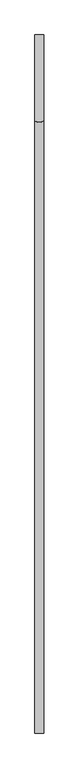
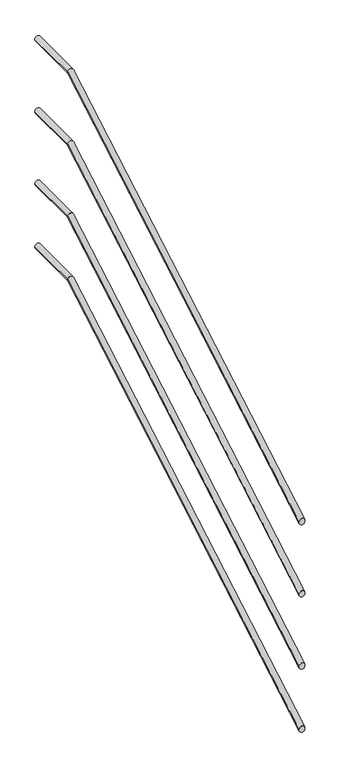
"""IFC4 building model written with IfcOpenShell, lengths in millimetres: railing geometry."""

from ifc_helpers import new_model, si_unit, frame, origin, place, context, project, spatial, circle_curve, ellipse_curve, source, transform, mapped, element, save
from ifc_brep_helpers import plane_surface, cylinder_surface, advanced_brep


def railing_3ea5c4bd(model_context):
    return source(origin(), model_context, "Body", "AdvancedBrep", [
        advanced_brep(
        [(-3259.6, 13399.5208589, 1336.7361432), (-3289.6, 13399.5208589, 1336.7361432), (-3259.6, 15503.5584173, 2557.9030398), (-3289.6, 15503.5584173, 2557.9030398), (-3259.6, 15799.5208589, 2557.9030398), (-3289.6, 15799.5208589, 2557.9030398)],
        [
            (0, 1, ellipse_curve(frame((-3274.6, 13399.5208589, 1336.7361432), z_axis=(0.0, -1.0, 0.0), x_axis=(0.0, 0.0, -1.0)), 17.3433672, 15.0)),
            (1, 0, ellipse_curve(frame((-3274.6, 13399.5208589, 1336.7361432), z_axis=(0.0, -1.0, 0.0), x_axis=(0.0, 0.0, -1.0)), 17.3433672, 15.0)),
            (0, 2),
            (2, 3, ellipse_curve(frame((-3274.6, 15503.5584173, 2557.9030398), z_axis=(0.0, -0.9656303515230847, -0.25991926480621574), x_axis=(0.0, 0.25991926480621586, -0.9656303515230849)), 15.5338945, 15.0)),
            (3, 1),
            (3, 2, ellipse_curve(frame((-3274.6, 15503.5584173, 2557.9030398), z_axis=(0.0, -0.9656303515230847, -0.25991926480621574), x_axis=(0.0, 0.25991926480621586, -0.9656303515230849)), 15.5338945, 15.0)),
            (4, 5, circle_curve(frame((-3274.6, 15799.5208589, 2557.9030398), z_axis=(0.0, 1.0, 0.0), x_axis=(-1.0, 0.0, 0.0)), 15.0)),
            (5, 4, circle_curve(frame((-3274.6, 15799.5208589, 2557.9030398), z_axis=(0.0, 1.0, 0.0), x_axis=(-1.0, 0.0, 0.0)), 15.0)),
            (2, 4),
            (5, 3),
        ],
        [
            plane_surface(frame((-3274.6, 13399.5208589, 1354.0795104), z_axis=(0.0, -1.0, 0.0), x_axis=(0.0, 0.0, 1.0))),
            cylinder_surface(frame((-3274.6, 13407.0504368, 1341.1062512), z_axis=(0.0, -0.8648839515651926, -0.5019718620848959), x_axis=(-1.0, 0.0, 0.0)), 15.0),
            plane_surface(frame((-3274.6, 15799.5208589, 2572.9030398), z_axis=(0.0, 1.0, 0.0), x_axis=(0.0, 0.0, 1.0))),
            cylinder_surface(frame((-3274.6, 15499.5208589, 2557.9030398), z_axis=(0.0, -1.0, 0.0), x_axis=(-1.0, 0.0, 0.0)), 15.0),
        ],
        [
            (0, [[1, 2]]),
            (1, [[-1, 3, 4, 5]]),
            (1, [[-2, -5, 6, -3]]),
            (2, [[7, 8]]),
            (3, [[-4, 9, -8, 10]]),
            (3, [[-6, -10, -7, -9]]),
        ],
    ),
        advanced_brep(
        [(-3259.6, 13399.5208589, 536.7361432), (-3289.6, 13399.5208589, 536.7361432), (-3259.6, 15503.5584173, 1757.9030398), (-3289.6, 15503.5584173, 1757.9030398), (-3259.6, 15799.5208589, 1757.9030398), (-3289.6, 15799.5208589, 1757.9030398)],
        [
            (0, 1, ellipse_curve(frame((-3274.6, 13399.5208589, 536.7361432), z_axis=(0.0, -1.0, 0.0), x_axis=(0.0, 0.0, -1.0)), 17.3433672, 15.0)),
            (1, 0, ellipse_curve(frame((-3274.6, 13399.5208589, 536.7361432), z_axis=(0.0, -1.0, 0.0), x_axis=(0.0, 0.0, -1.0)), 17.3433672, 15.0)),
            (0, 2),
            (2, 3, ellipse_curve(frame((-3274.6, 15503.5584173, 1757.9030398), z_axis=(0.0, -0.9656303515230847, -0.25991926480621574), x_axis=(0.0, 0.25991926480621586, -0.9656303515230849)), 15.5338945, 15.0)),
            (3, 1),
            (3, 2, ellipse_curve(frame((-3274.6, 15503.5584173, 1757.9030398), z_axis=(0.0, -0.9656303515230847, -0.25991926480621574), x_axis=(0.0, 0.25991926480621586, -0.9656303515230849)), 15.5338945, 15.0)),
            (4, 5, circle_curve(frame((-3274.6, 15799.5208589, 1757.9030398), z_axis=(0.0, 1.0, 0.0), x_axis=(-1.0, 0.0, 0.0)), 15.0)),
            (5, 4, circle_curve(frame((-3274.6, 15799.5208589, 1757.9030398), z_axis=(0.0, 1.0, 0.0), x_axis=(-1.0, 0.0, 0.0)), 15.0)),
            (2, 4),
            (5, 3),
        ],
        [
            plane_surface(frame((-3274.6, 13399.5208589, 554.0795104), z_axis=(0.0, -1.0, 0.0), x_axis=(0.0, 0.0, 1.0))),
            cylinder_surface(frame((-3274.6, 13407.0504368, 541.1062512), z_axis=(0.0, -0.8648839515651926, -0.5019718620848959), x_axis=(-1.0, 0.0, 0.0)), 15.0),
            plane_surface(frame((-3274.6, 15799.5208589, 1772.9030398), z_axis=(0.0, 1.0, 0.0), x_axis=(0.0, 0.0, 1.0))),
            cylinder_surface(frame((-3274.6, 15499.5208589, 1757.9030398), z_axis=(0.0, -1.0, 0.0), x_axis=(-1.0, 0.0, 0.0)), 15.0),
        ],
        [
            (0, [[1, 2]]),
            (1, [[-1, 3, 4, 5]]),
            (1, [[-2, -5, 6, -3]]),
            (2, [[7, 8]]),
            (3, [[-4, 9, -8, 10]]),
            (3, [[-6, -10, -7, -9]]),
        ],
    ),
        advanced_brep(
        [(-3259.6, 13399.5208589, 936.7361432), (-3289.6, 13399.5208589, 936.7361432), (-3259.6, 15503.5584173, 2157.9030398), (-3289.6, 15503.5584173, 2157.9030398), (-3259.6, 15799.5208589, 2157.9030398), (-3289.6, 15799.5208589, 2157.9030398)],
        [
            (0, 1, ellipse_curve(frame((-3274.6, 13399.5208589, 936.7361432), z_axis=(0.0, -1.0, 0.0), x_axis=(0.0, 0.0, -1.0)), 17.3433672, 15.0)),
            (1, 0, ellipse_curve(frame((-3274.6, 13399.5208589, 936.7361432), z_axis=(0.0, -1.0, 0.0), x_axis=(0.0, 0.0, -1.0)), 17.3433672, 15.0)),
            (0, 2),
            (2, 3, ellipse_curve(frame((-3274.6, 15503.5584173, 2157.9030398), z_axis=(0.0, -0.9656303515230847, -0.25991926480621574), x_axis=(0.0, 0.25991926480621586, -0.9656303515230849)), 15.5338945, 15.0)),
            (3, 1),
            (3, 2, ellipse_curve(frame((-3274.6, 15503.5584173, 2157.9030398), z_axis=(0.0, -0.9656303515230847, -0.25991926480621574), x_axis=(0.0, 0.25991926480621586, -0.9656303515230849)), 15.5338945, 15.0)),
            (4, 5, circle_curve(frame((-3274.6, 15799.5208589, 2157.9030398), z_axis=(0.0, 1.0, 0.0), x_axis=(-1.0, 0.0, 0.0)), 15.0)),
            (5, 4, circle_curve(frame((-3274.6, 15799.5208589, 2157.9030398), z_axis=(0.0, 1.0, 0.0), x_axis=(-1.0, 0.0, 0.0)), 15.0)),
            (2, 4),
            (5, 3),
        ],
        [
            plane_surface(frame((-3274.6, 13399.5208589, 954.0795104), z_axis=(0.0, -1.0, 0.0), x_axis=(0.0, 0.0, 1.0))),
            cylinder_surface(frame((-3274.6, 13407.0504368, 941.1062512), z_axis=(0.0, -0.8648839515651926, -0.5019718620848959), x_axis=(-1.0, 0.0, 0.0)), 15.0),
            plane_surface(frame((-3274.6, 15799.5208589, 2172.9030398), z_axis=(0.0, 1.0, 0.0), x_axis=(0.0, 0.0, 1.0))),
            cylinder_surface(frame((-3274.6, 15499.5208589, 2157.9030398), z_axis=(0.0, -1.0, 0.0), x_axis=(-1.0, 0.0, 0.0)), 15.0),
        ],
        [
            (0, [[1, 2]]),
            (1, [[-1, 3, 4, 5]]),
            (1, [[-2, -5, 6, -3]]),
            (2, [[7, 8]]),
            (3, [[-4, 9, -8, 10]]),
            (3, [[-6, -10, -7, -9]]),
        ],
    ),
        advanced_brep(
        [(-3259.6, 13399.5208589, 186.7361432), (-3289.6, 13399.5208589, 186.7361432), (-3259.6, 15503.5584173, 1407.9030398), (-3289.6, 15503.5584173, 1407.9030398), (-3259.6, 15799.5208589, 1407.9030398), (-3289.6, 15799.5208589, 1407.9030398)],
        [
            (0, 1, ellipse_curve(frame((-3274.6, 13399.5208589, 186.7361432), z_axis=(0.0, -1.0, 0.0), x_axis=(0.0, 0.0, -1.0)), 17.3433672, 15.0)),
            (1, 0, ellipse_curve(frame((-3274.6, 13399.5208589, 186.7361432), z_axis=(0.0, -1.0, 0.0), x_axis=(0.0, 0.0, -1.0)), 17.3433672, 15.0)),
            (0, 2),
            (2, 3, ellipse_curve(frame((-3274.6, 15503.5584173, 1407.9030398), z_axis=(0.0, -0.9656303515230847, -0.25991926480621574), x_axis=(0.0, 0.25991926480621586, -0.9656303515230849)), 15.5338945, 15.0)),
            (3, 1),
            (3, 2, ellipse_curve(frame((-3274.6, 15503.5584173, 1407.9030398), z_axis=(0.0, -0.9656303515230847, -0.25991926480621574), x_axis=(0.0, 0.25991926480621586, -0.9656303515230849)), 15.5338945, 15.0)),
            (4, 5, circle_curve(frame((-3274.6, 15799.5208589, 1407.9030398), z_axis=(0.0, 1.0, 0.0), x_axis=(-1.0, 0.0, 0.0)), 15.0)),
            (5, 4, circle_curve(frame((-3274.6, 15799.5208589, 1407.9030398), z_axis=(0.0, 1.0, 0.0), x_axis=(-1.0, 0.0, 0.0)), 15.0)),
            (2, 4),
            (5, 3),
        ],
        [
            plane_surface(frame((-3274.6, 13399.5208589, 204.0795104), z_axis=(0.0, -1.0, 0.0), x_axis=(0.0, 0.0, 1.0))),
            cylinder_surface(frame((-3274.6, 13407.0504368, 191.1062512), z_axis=(0.0, -0.8648839515651926, -0.5019718620848959), x_axis=(-1.0, 0.0, 0.0)), 15.0),
            plane_surface(frame((-3274.6, 15799.5208589, 1422.9030398), z_axis=(0.0, 1.0, 0.0), x_axis=(0.0, 0.0, 1.0))),
            cylinder_surface(frame((-3274.6, 15499.5208589, 1407.9030398), z_axis=(0.0, -1.0, 0.0), x_axis=(-1.0, 0.0, 0.0)), 15.0),
        ],
        [
            (0, [[1, 2]]),
            (1, [[-1, 3, 4, 5]]),
            (1, [[-2, -5, 6, -3]]),
            (2, [[7, 8]]),
            (3, [[-4, 9, -8, 10]]),
            (3, [[-6, -10, -7, -9]]),
        ],
    ),
    ])


if __name__ == "__main__":
    model = new_model("IFC4")
    model_context = context("Model", 3, world=origin())
    ifc_project = project(units=[si_unit("LENGTHUNIT", "METRE", prefix="MILLI")], contexts=[model_context])
    site = spatial("IfcSite", under=ifc_project)
    building = spatial("IfcBuilding", under=site)
    placement = place(None, origin())
    railing_shape = railing_3ea5c4bd(model_context)
    element("IfcRailing", 1, at=placement, inside=building, context=model_context, shape_type="MappedRepresentation", body=[
        mapped(railing_shape, transform((0.0, 0.0, 0.0), x_axis=(1.0, 0.0, 0.0), y_axis=(0.0, 1.0, 0.0), z_axis=(0.0, 0.0, 1.0))),
    ])
    save(model, "model.ifc")
